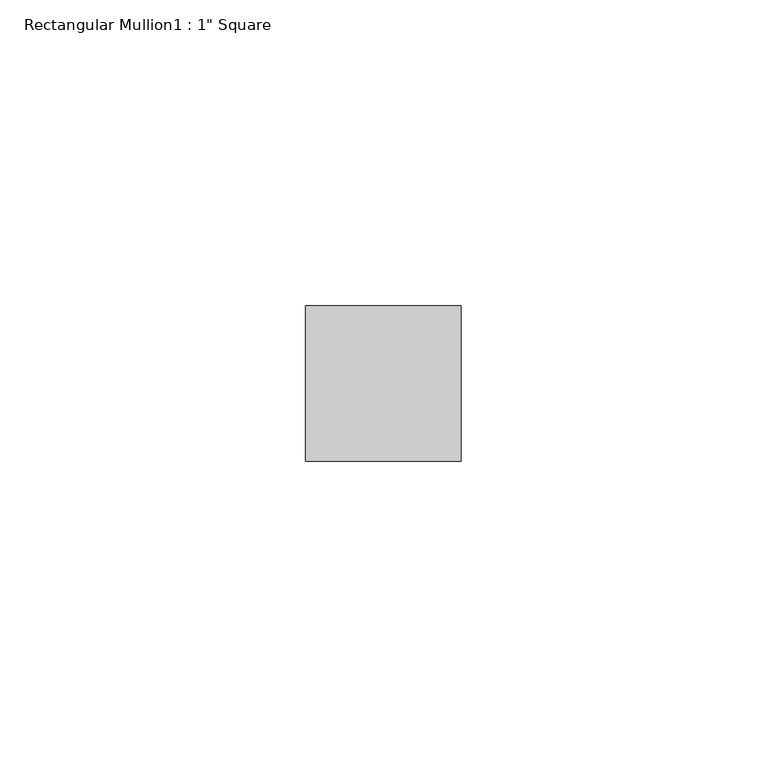
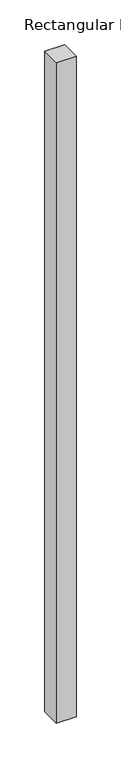
"""IFC4 building model written with IfcOpenShell, lengths in millimetres: member geometry."""

import ifcopenshell
import ifcopenshell.guid

model = None  # the IFC model being written
_history = None  # IfcOwnerHistory: only IFC2X3 demands one
_inside = {}  # id of a spatial element -> (the spatial element, [elements in it])
_under = {}  # id of a project, library or spatial element -> (it, [spatial elements below it])
_declared = {}  # id of a project -> (the project, [libraries it declares])
_typed = {}  # id of a type object -> (the type object, [elements of that type])
_made_of = {}  # id of a material, layer set ... -> (it, [elements and type objects made of it])


def new_model(schema):
    """Start an empty IFC model of exactly this schema.

    Asked for "IFC4X3", IfcOpenShell would pick the latest addendum, in which some entities
    have other attributes; the version numbers below select the first issue.
    IFC2X3 requires an IfcOwnerHistory on every rooted entity: one is made here for all.
    """
    global model, _history
    if schema == "IFC4X3":
        model = ifcopenshell.file(schema_version=(4, 3, 0, 0))
    else:
        model = ifcopenshell.file(schema=schema)
    _inside.clear()
    _under.clear()
    _declared.clear()
    _typed.clear()
    _made_of.clear()
    _history = None
    if model.schema == "IFC2X3":
        org = make("IfcOrganization", Name="unknown")
        user = make(
            "IfcPersonAndOrganization",
            ThePerson=make("IfcPerson", FamilyName="unknown"),
            TheOrganization=org,
        )
        app = make(
            "IfcApplication",
            ApplicationDeveloper=org,
            Version="unknown",
            ApplicationFullName="unknown",
            ApplicationIdentifier="unknown",
        )
        _history = make(
            "IfcOwnerHistory",
            OwningUser=user,
            OwningApplication=app,
            ChangeAction="ADDED",
            CreationDate=0,
        )
    return model


def make(cls, **values):
    """One entity of the class cls with the attributes given. An attribute that is None is left unset."""
    return model.create_entity(
        cls, **{name: value for name, value in values.items() if value is not None}
    )


def rooted(cls, **values):
    """An entity with a GlobalId (a new one), such as an element, a storey or a relation."""
    return make(cls, GlobalId=ifcopenshell.guid.new(), OwnerHistory=_history, **values)


def si_unit(unit_type, name, prefix=None):
    """IfcSIUnit, for example si_unit("LENGTHUNIT", "METRE", prefix="MILLI")."""
    return make("IfcSIUnit", UnitType=unit_type, Prefix=prefix, Name=name)


def assignment(units):
    """IfcUnitAssignment: the units of a project."""
    return None if units is None else make("IfcUnitAssignment", Units=units)


def point(xyz):
    """IfcCartesianPoint."""
    return None if xyz is None else make("IfcCartesianPoint", Coordinates=xyz)


def direction(xyz):
    """IfcDirection."""
    return None if xyz is None else make("IfcDirection", DirectionRatios=xyz)


def frame(location, z_axis=None, x_axis=None):
    """IfcAxis2Placement3D, a coordinate frame: its origin and axes. An axis left out is left unset."""
    return make(
        "IfcAxis2Placement3D",
        Location=point(location),
        Axis=direction(z_axis),
        RefDirection=direction(x_axis),
    )


def origin():
    """The frame at (0, 0, 0) with its axes left unset."""
    return frame((0.0, 0.0, 0.0))


def place(relative_to, where):
    """IfcLocalPlacement: puts the frame where relative to a parent placement (None: the world)."""
    return make(
        "IfcLocalPlacement", PlacementRelTo=relative_to, RelativePlacement=where
    )


def context(
    kind, dimensions, precision=None, world=None, true_north=None, identifier=None
):
    """IfcGeometricRepresentationContext, for example the 3D "Model" context."""
    return make(
        "IfcGeometricRepresentationContext",
        ContextIdentifier=identifier,
        ContextType=kind,
        CoordinateSpaceDimension=dimensions,
        Precision=precision,
        WorldCoordinateSystem=world,
        TrueNorth=true_north,
    )


def project(units=None, contexts=None):
    """IfcProject with its units and contexts."""
    return rooted(
        "IfcProject",
        Name="project",
        RepresentationContexts=contexts,
        UnitsInContext=assignment(units),
    )


def spatial(cls, under=None, at=None, **own):
    """A site, building, storey or space (cls), placed at a placement, below another one or the project."""
    s = rooted(cls, ObjectPlacement=at, **own)
    if under is not None:
        _under.setdefault(under.id(), (under, []))[1].append(s)
    return s


def polyline(points):
    """IfcPolyline through the points."""
    return make("IfcPolyline", Points=[point(p) for p in points])


def outline(outer, holes=None, kind="AREA"):
    """IfcArbitraryClosedProfileDef: a profile drawn as a closed curve; with holes, ...WithVoids."""
    if holes is None:
        return make("IfcArbitraryClosedProfileDef", ProfileType=kind, OuterCurve=outer)
    return make(
        "IfcArbitraryProfileDefWithVoids",
        ProfileType=kind,
        OuterCurve=outer,
        InnerCurves=holes,
    )


def extrude(swept, where, along, depth):
    """IfcExtrudedAreaSolid: the profile swept, set in the frame where, extruded along a direction by depth."""
    return make(
        "IfcExtrudedAreaSolid",
        SweptArea=swept,
        Position=where,
        ExtrudedDirection=direction(along),
        Depth=depth,
    )


def shape(context_of_items, identifier, shape_type, items):
    """IfcShapeRepresentation: the items that make up one representation, for example the "Body"."""
    return make(
        "IfcShapeRepresentation",
        ContextOfItems=context_of_items,
        RepresentationIdentifier=identifier,
        RepresentationType=shape_type,
        Items=items,
    )


def source(mapping_origin, context_of_items, identifier, shape_type, items):
    """IfcRepresentationMap: a shape defined once, which mapped items show again and again."""
    return make(
        "IfcRepresentationMap",
        MappingOrigin=mapping_origin,
        MappedRepresentation=shape(context_of_items, identifier, shape_type, items),
    )


def transform(
    local_origin,
    x_axis=None,
    y_axis=None,
    z_axis=None,
    scale=None,
    scale2=None,
    scale3=None,
    uniform=True,
):
    """IfcCartesianTransformationOperator3D, or its non-uniform kind. x_axis, y_axis, z_axis: its Axis1, 2, 3."""
    if uniform:
        return make(
            "IfcCartesianTransformationOperator3D",
            Axis1=direction(x_axis),
            Axis2=direction(y_axis),
            LocalOrigin=point(local_origin),
            Scale=scale,
            Axis3=direction(z_axis),
        )
    return make(
        "IfcCartesianTransformationOperator3DnonUniform",
        Axis1=direction(x_axis),
        Axis2=direction(y_axis),
        LocalOrigin=point(local_origin),
        Scale=scale,
        Axis3=direction(z_axis),
        Scale2=scale2,
        Scale3=scale3,
    )


def mapped(mapping_source, mapping_target):
    """IfcMappedItem: shows the shape of a source again, moved by a transform."""
    return make(
        "IfcMappedItem", MappingSource=mapping_source, MappingTarget=mapping_target
    )


def made_of(thing, what):
    """Note that an element or type object is made of a material, layer set ...; save() writes the relation."""
    if what is not None:
        _made_of.setdefault(what.id(), (what, []))[1].append(thing)
    return thing


def element(
    cls,
    number,
    at=None,
    inside=None,
    cuts=None,
    type_object=None,
    material=None,
    context=None,
    identifier="Body",
    shape_type=None,
    held_by="IfcProductDefinitionShape",
    body=None,
    shapes=None,
    **own,
):
    """One element of the class cls, such as IfcWall. Its Tag is "e" and its number.

    at: its placement. inside: the storey or other place that contains it. cuts: it is an
    opening in that element (IfcRelVoidsElement). A single representation is given by context,
    identifier, shape_type and body (its items); several are given by shapes. held_by: the class
    of the entity that holds the representations. save() writes the other relations.
    """
    e = rooted(cls, Tag="e%d" % number, ObjectPlacement=at, **own)
    if body is not None:
        shapes = [shape(context, identifier, shape_type, body)]
    if shapes is not None:
        e.Representation = make(held_by, Representations=shapes)
    if inside is not None:
        _inside.setdefault(inside.id(), (inside, []))[1].append(e)
    if cuts is not None:
        rooted(
            "IfcRelVoidsElement", RelatingBuildingElement=cuts, RelatedOpeningElement=e
        )
    if type_object is not None:
        _typed.setdefault(type_object.id(), (type_object, []))[1].append(e)
    return made_of(e, material)


def aggregate(whole, parts):
    """IfcRelAggregates: a whole, such as a stair, and the parts it consists of."""
    return rooted("IfcRelAggregates", RelatingObject=whole, RelatedObjects=parts)


def save(model, path):
    """Write the relations noted so far, then the file.

    IfcRelAggregates (storeys below a building ...), IfcRelContainedInSpatialStructure (elements
    in a storey), IfcRelDefinesByType, IfcRelAssociatesMaterial and IfcRelDeclares: one each for
    every whole, place, type object, material and project.
    """
    for whole, parts in _under.values():
        aggregate(whole, parts)
    for where, things in _inside.values():
        rooted(
            "IfcRelContainedInSpatialStructure",
            RelatedElements=things,
            RelatingStructure=where,
        )
    for kind, things in _typed.values():
        rooted("IfcRelDefinesByType", RelatedObjects=things, RelatingType=kind)
    for what, things in _made_of.values():
        rooted("IfcRelAssociatesMaterial", RelatedObjects=things, RelatingMaterial=what)
    for by, libraries in _declared.values():
        rooted("IfcRelDeclares", RelatingContext=by, RelatedDefinitions=libraries)
    model.write(path)


def member_48a22cbc(model_context):
    return source(origin(), model_context, "Body", "SweptSolid", [
        extrude(outline(polyline([(0.0, -19.05), (0.0, -44.45), (-25.4, -44.45), (-25.4, -19.05), (0.0, -19.05)])), frame((0.0, 0.0, -897.3298256), z_axis=(0.0, 0.0, 1.0), x_axis=(1.0, 0.0, 0.0)), (0.0, 0.0, 1.0), 897.3298256),
    ])


if __name__ == "__main__":
    model = new_model("IFC4")
    model_context = context("Model", 3, world=origin())
    ifc_project = project(units=[si_unit("LENGTHUNIT", "METRE", prefix="MILLI")], contexts=[model_context])
    site = spatial("IfcSite", under=ifc_project)
    building = spatial("IfcBuilding", under=site)
    placement = place(None, origin())
    member_shape = member_48a22cbc(model_context)
    element("IfcMember", 1, ObjectType="Rectangular Mullion1 : 1\" Square", at=placement, inside=building, context=model_context, shape_type="MappedRepresentation", body=[
        mapped(member_shape, transform((0.0, 0.0, 0.0), x_axis=(1.0, 0.0, 0.0), y_axis=(0.0, 1.0, 0.0), z_axis=(0.0, 0.0, 1.0))),
    ])
    save(model, "model.ifc")

# Revit data of these elements
# Type "Rectangular Mullion1 : 1\" Square"
#   built-in parameter 1007351 = 0.104167 (stored number, unit not read)
#   built-in parameter 1007304 = 0.0833333 (stored number, unit not read)
#   built-in parameter 1007301 = 0.0416667 (stored number, unit not read)
#   built-in parameter 1007300 = 0.0416667 (stored number, unit not read)
